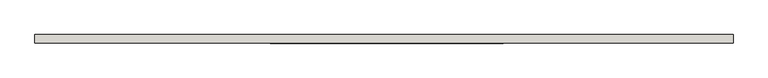
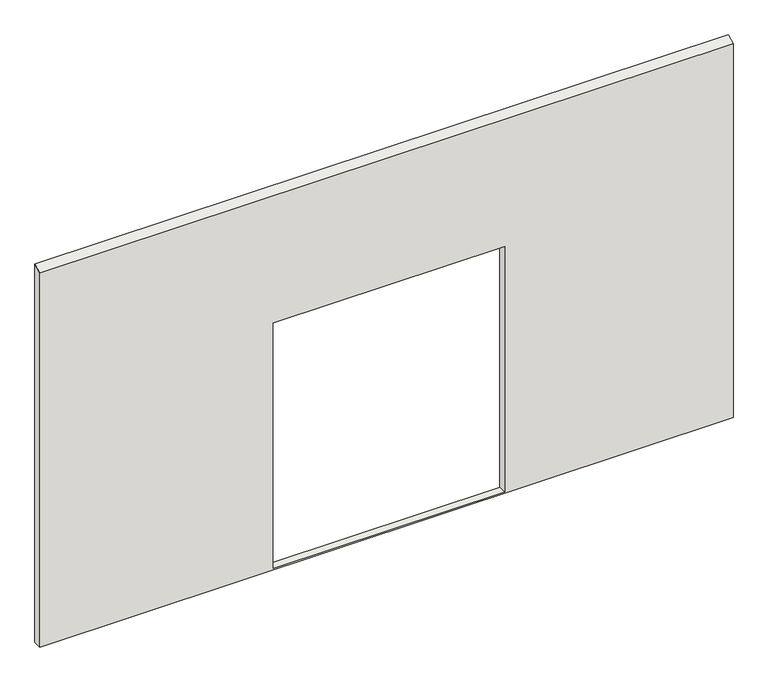
"""IFC4 building model written with IfcOpenShell, lengths in millimetres: wall geometry, 0_3d_modell."""

from ifc_helpers import new_model, si_unit, origin, place, context, project, spatial, faceted_brep, source, transform, mapped, element, save


def wall_0d87ef2e(model_context):
    return source(origin(), model_context, "Body", "Brep", [
        faceted_brep([(1919.0, 70.0, 10.0), (1919.0, 70.0, 2145.0), (1919.0, 0.0, 2145.0), (1919.0, 0.0, 10.0), (3819.0, 70.0, 2145.0), (3819.0, 0.0, 2145.0), (3819.0, 70.0, 10.0), (3819.0, 0.0, 10.0), (5694.0, 0.0, 3247.913011), (5694.0, 70.0, 3283.5797924), (0.0, 70.0, 3283.5797924), (0.0, 0.0, 3247.913011), (0.0, 70.0, 0.0), (0.0, 0.0, 0.0), (5694.0, 0.0, 0.0), (5694.0, 70.0, 0.0)], [[[0, 1, 2, 3]], [[1, 4, 5, 2]], [[4, 6, 7, 5]], [[6, 0, 3, 7]], [[8, 9, 10, 11]], [[11, 10, 12, 13]], [[9, 8, 14, 15]], [[8, 11, 13, 14], [3, 2, 5, 7]], [[15, 12, 10, 9], [1, 0, 6, 4]], [[12, 15, 14, 13]]]),
    ])


if __name__ == "__main__":
    model = new_model("IFC4")
    model_context = context("Model", 3, world=origin())
    ifc_project = project(units=[si_unit("LENGTHUNIT", "METRE", prefix="MILLI")], contexts=[model_context])
    site = spatial("IfcSite", under=ifc_project)
    building = spatial("IfcBuilding", under=site)
    placement = place(None, origin())
    wall_shape = wall_0d87ef2e(model_context)
    element("IfcWall", 1, ObjectType="0_3d_modell", at=placement, inside=building, context=model_context, shape_type="MappedRepresentation", body=[
        mapped(wall_shape, transform((0.0, 0.0, 0.0), x_axis=(1.0, 0.0, 0.0), y_axis=(0.0, 1.0, 0.0), z_axis=(0.0, 0.0, 1.0))),
    ])
    save(model, "model.ifc")

# Revit data of these elements
# Element 1 (IfcWall, "0_3d_modell")
#   Materials on its faces: "Glass_Simple"
# Materials
#   "Glass_Simple": class "Unassigned", colour RGB 255 255 255, transparency 0.9
